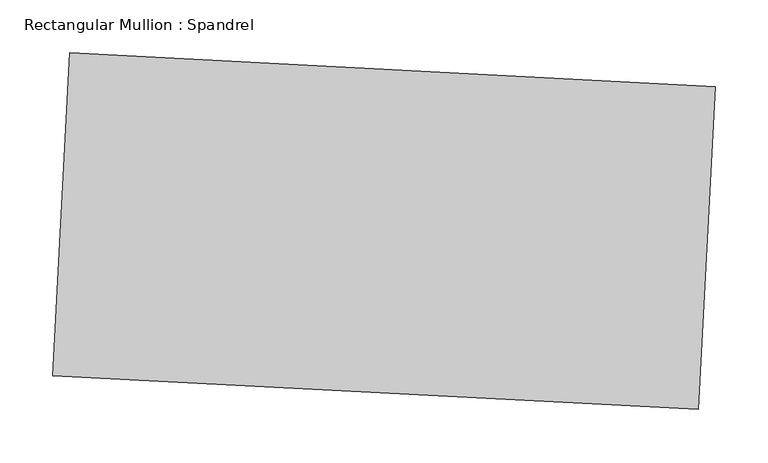
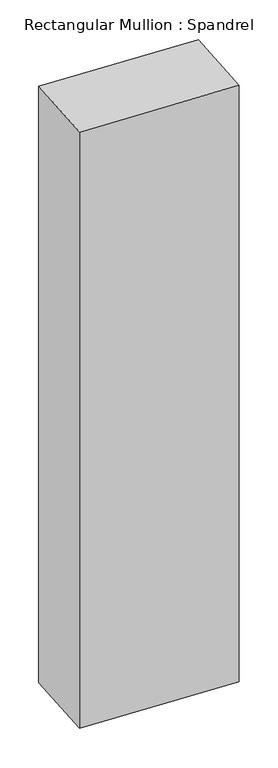
"""IFC4 building model written with IfcOpenShell, lengths in millimetres: member geometry, Rectangular Mullion : Spandrel."""

from ifc_helpers import new_model, si_unit, frame, origin, place, context, project, spatial, polyline, outline, extrude, source, transform, mapped, element, save


def rectangular_mullion_spandrel_31a1125c(model_context):
    return source(origin(), model_context, "Body", "SweptSolid", [
        extrude(outline(polyline([(312.3582819, 136.2391416), (296.4062825, -168.1431406), (-312.3582819, -136.2391416), (-296.4062825, 168.1431406), (312.3582819, 136.2391416)])), frame((0.0, 0.0, -2475.9433652), z_axis=(0.0, 0.0, 1.0), x_axis=(1.0, 0.0, 0.0)), (0.0, 0.0, 1.0), 2475.9433652),
    ])


if __name__ == "__main__":
    model = new_model("IFC4")
    model_context = context("Model", 3, world=origin())
    ifc_project = project(units=[si_unit("LENGTHUNIT", "METRE", prefix="MILLI")], contexts=[model_context])
    site = spatial("IfcSite", under=ifc_project)
    building = spatial("IfcBuilding", under=site)
    placement = place(None, origin())
    rectangular_mullion_spandrel_shape = rectangular_mullion_spandrel_31a1125c(model_context)
    element("IfcMember", 1, ObjectType="Rectangular Mullion : Spandrel", at=placement, inside=building, context=model_context, shape_type="MappedRepresentation", body=[
        mapped(rectangular_mullion_spandrel_shape, transform((0.0, 0.0, 0.0), x_axis=(1.0, 0.0, 0.0), y_axis=(0.0, 1.0, 0.0), z_axis=(0.0, 0.0, 1.0))),
    ])
    save(model, "model.ifc")

# Revit data of these elements
# Type "Rectangular Mullion : Spandrel"
#   built-in parameter 1007304 = 1 (stored number, unit not read)
#   built-in parameter 1007301 = 1 (stored number, unit not read)
#   built-in parameter 1007300 = 1 (stored number, unit not read)
# Element 1 (IfcMember, "Rectangular Mullion : Spandrel")
#   Materials on its faces: "Aluminum"
# Materials
#   "Aluminum": class "Metal", colour RGB 247 247 247, transparency 0, Description = "Aluminum 6061", Cost = 0
